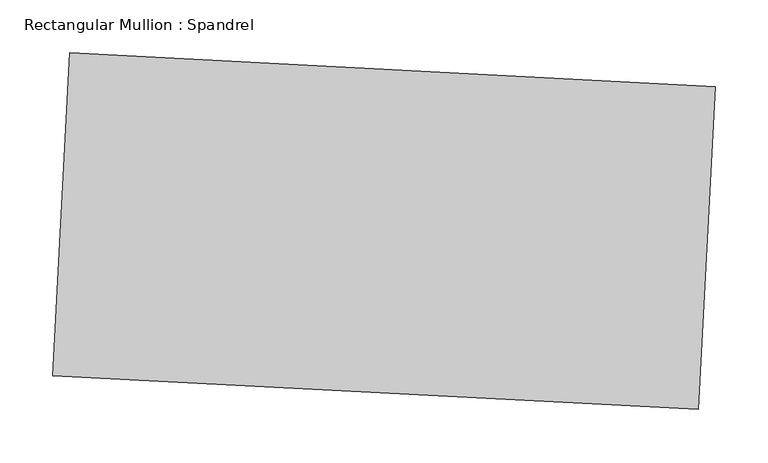
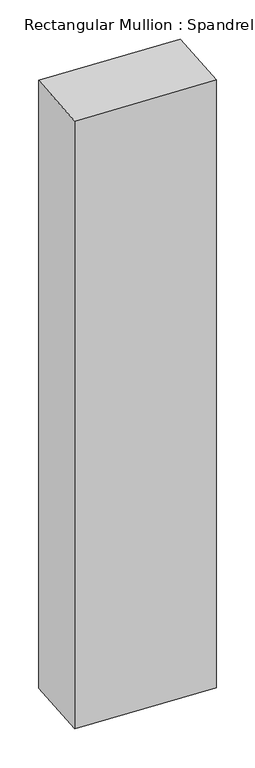
"""IFC4 building model written with IfcOpenShell, lengths in millimetres: member geometry, Rectangular Mullion : Spandrel."""

from ifc_helpers import new_model, si_unit, frame, origin, place, context, project, spatial, polyline, outline, extrude, source, transform, mapped, element, save


def rectangular_mullion_spandrel_ffee690b(model_context):
    return source(origin(), model_context, "Body", "SweptSolid", [
        extrude(outline(polyline([(7.5582819, 136.2391416), (-8.3937175, -168.1431406), (-617.1582819, -136.2391416), (-601.2062825, 168.1431406), (7.5582819, 136.2391416)])), frame((0.0, 0.0, -2845.3134854), z_axis=(0.0, 0.0, 1.0), x_axis=(1.0, 0.0, 0.0)), (0.0, 0.0, 1.0), 2845.3134854),
    ])


if __name__ == "__main__":
    model = new_model("IFC4")
    model_context = context("Model", 3, world=origin())
    ifc_project = project(units=[si_unit("LENGTHUNIT", "METRE", prefix="MILLI")], contexts=[model_context])
    site = spatial("IfcSite", under=ifc_project)
    building = spatial("IfcBuilding", under=site)
    placement = place(None, origin())
    rectangular_mullion_spandrel_shape = rectangular_mullion_spandrel_ffee690b(model_context)
    element("IfcMember", 1, ObjectType="Rectangular Mullion : Spandrel", at=placement, inside=building, context=model_context, shape_type="MappedRepresentation", body=[
        mapped(rectangular_mullion_spandrel_shape, transform((0.0, 0.0, 0.0), x_axis=(1.0, 0.0, 0.0), y_axis=(0.0, 1.0, 0.0), z_axis=(0.0, 0.0, 1.0))),
    ])
    save(model, "model.ifc")

# Revit data of these elements
# Type "Rectangular Mullion : Spandrel"
#   built-in parameter 1007304 = 1 (stored number, unit not read)
#   built-in parameter 1007301 = 1 (stored number, unit not read)
#   built-in parameter 1007300 = 1 (stored number, unit not read)
# Element 1 (IfcMember, "Rectangular Mullion : Spandrel")
#   Materials on its faces: "Aluminum"
# Materials
#   "Aluminum": class "Metal", colour RGB 247 247 247, transparency 0, Description = "Aluminum 6061", Cost = 0
